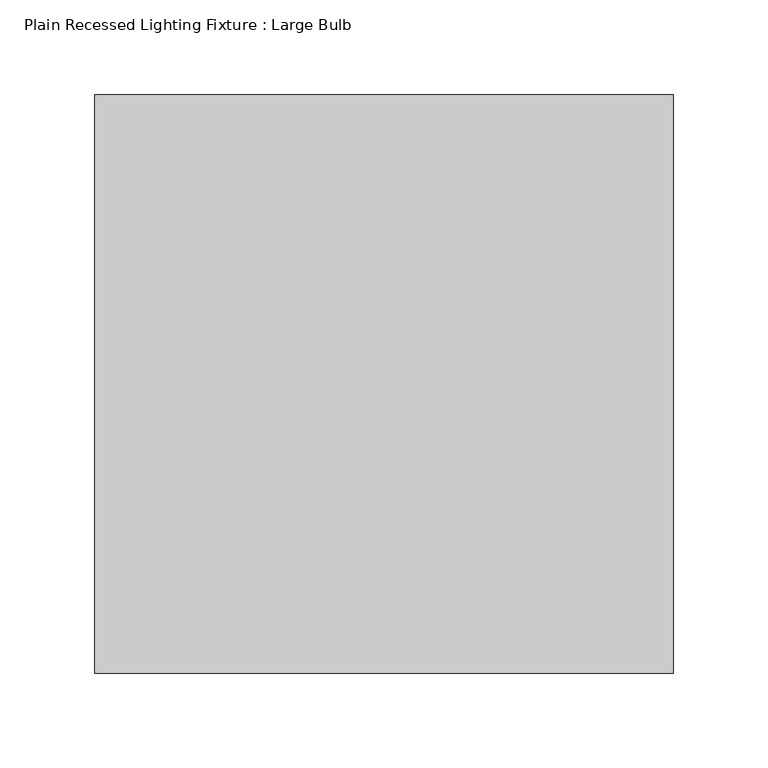
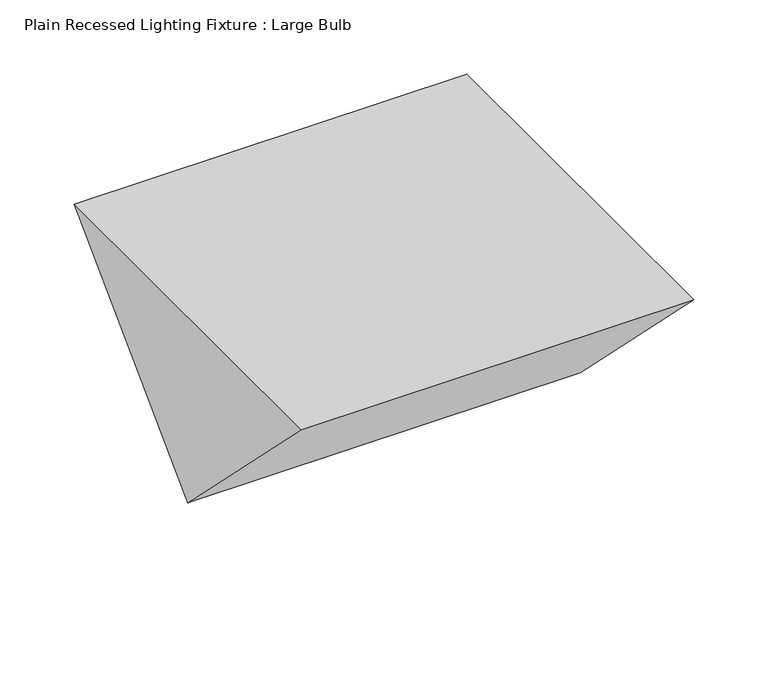
"""IFC4 building model written with IfcOpenShell, lengths in millimetres: light fixture geometry, Plain Recessed Lighting Fixture : Large Bulb."""

from ifc_helpers import new_model, si_unit, frame, origin, place, context, project, spatial, polyline, outline, extrude, source, transform, mapped, element, save


def plain_recessed_lighting_fixture_large_bulb_b9741ada(model_context):
    return source(origin(), model_context, "Body", "SweptSolid", [
        extrude(outline(polyline([(-304.8, 0.0), (0.0, 0.0), (-152.4, -152.4), (-304.8, 0.0)])), frame((0.0, 0.0, 0.0), z_axis=(1.0, 0.0, 0.0), x_axis=(0.0, 1.0, 0.0)), (0.0, 0.0, 1.0), 304.8),
    ])


if __name__ == "__main__":
    model = new_model("IFC4")
    model_context = context("Model", 3, world=origin())
    ifc_project = project(units=[si_unit("LENGTHUNIT", "METRE", prefix="MILLI")], contexts=[model_context])
    site = spatial("IfcSite", under=ifc_project)
    building = spatial("IfcBuilding", under=site)
    placement = place(None, origin())
    plain_recessed_lighting_fixture_large_bulb_shape = plain_recessed_lighting_fixture_large_bulb_b9741ada(model_context)
    element("IfcLightFixture", 1, ObjectType="Plain Recessed Lighting Fixture : Large Bulb", at=placement, inside=building, context=model_context, shape_type="MappedRepresentation", body=[
        mapped(plain_recessed_lighting_fixture_large_bulb_shape, transform((0.0, 0.0, 0.0), x_axis=(1.0, 0.0, 0.0), y_axis=(0.0, 1.0, 0.0), z_axis=(0.0, 0.0, 1.0))),
    ])
    save(model, "model.ifc")

# Revit data of these elements
# Type "Plain Recessed Lighting Fixture : Large Bulb"
#   Photometric Web File = "2x22UA12.ies"
#   Width = 1' - 0"
#   Wattage = 62 W
#   built-in parameter 1150110 = 1 (stored number, unit not read)
#   built-in parameter 1150109 = 1 (stored number, unit not read)
#   built-in parameter 1150113 = 1 (stored number, unit not read)
#   Tilt Angle = -90.00°
#   Lumens = 5199.94 lm
#   built-in parameter 1114217 = 0.88 (stored number, unit not read)
#   built-in parameter 1150115 = 1 (stored number, unit not read)
#   built-in parameter 1150105 = 413.798 (stored number, unit not read)
#   Length = 1' - 0"
#   built-in parameter 1150112 = 1 (stored number, unit not read)
#   built-in parameter 1150114 = 1 (stored number, unit not read)
#   built-in parameter 1150107 = 4230 (stored number, unit not read)
#   built-in parameter 1150106 = 4.13798 (stored number, unit not read)
#   Emit from Rectangle Width = 1' - 0"
#   Emit from Rectangle Length = 1' - 0"
#   built-in parameter 1150104 = 7.79178 (stored number, unit not read)
#   Depth = 0' - 6"
#   Default Elevation = 4' - 0"
#   Ballast Voltage = 120 V
#   built-in parameter 1114218 = 0.88 (stored number, unit not read)
#   built-in parameter 1150133 = 10 (stored number, unit not read)
#   Apparent Load = 62 VA
#   built-in parameter 1150134 = 8
#   built-in parameter 1150137 = 1
#   Color Filter = 16777215
#   built-in parameter 1140040 [instance default] = 1
#   Load Classification = Lighting - Dwelling Unit
#   Emit Shape Visible in Rendering = no
#   Dimming Lamp Color Temperature Shift = (empty or 0)
#   Assembly Code = ""
